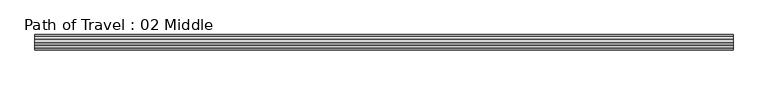
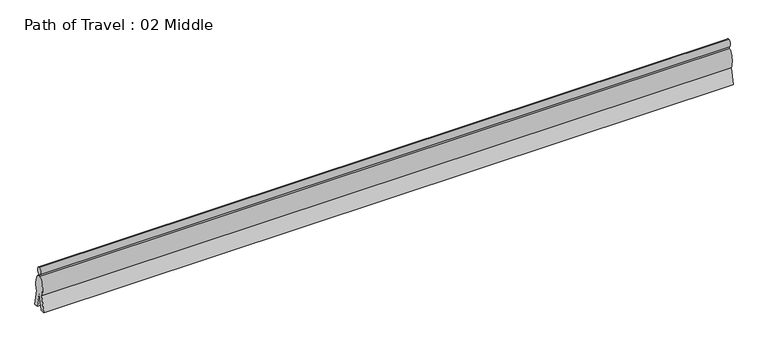
"""IFC4 building model written with IfcOpenShell, lengths in millimetres: proxy geometry, Path of Travel : 02 Middle."""

from ifc_helpers import new_model, si_unit, point, frame, origin, place, context, project, spatial, ellipse_curve, trimmed, source, transform, mapped, element, save
from ifc_brep_helpers import plane_surface, extruded_surface, advanced_brep


def path_of_travel_02_middle_70bd03b1(model_context):
    return source(origin(), model_context, "Body", "AdvancedBrep", [
        advanced_brep(
        [(227.5554837, 0.0, 1727.2), (227.5554837, 42.9018657, 1436.6534209), (227.5554837, 42.9018657, 1363.4763406), (227.5554837, 184.1186263, 643.4144547), (227.5554837, 297.5699544, 0.0), (227.5554837, 145.6574193, 0.0), (227.5554837, 0.0, 584.2), (227.5554837, -145.6574193, 0.0), (227.5554837, -297.5699544, 0.0), (227.5554837, -184.1186263, 643.4144547), (227.5554837, -42.9018657, 1363.4763406), (227.5554837, -42.9018657, 1436.6534209), (27507.1554837, 0.0, 1727.2), (27507.1554837, -42.9018657, 1436.6534209), (27507.1554837, -42.9018657, 1363.4763406), (27507.1554837, -184.1186263, 643.4144547), (27507.1554837, -297.5699544, 0.0), (27507.1554837, -145.6574193, 0.0), (27507.1554837, 0.0, 584.2), (27507.1554837, 145.6574193, 0.0), (27507.1554837, 297.5699544, 0.0), (27507.1554837, 184.1186263, 643.4144547), (27507.1554837, 42.9018657, 1363.4763406), (27507.1554837, 42.9018657, 1436.6534209)],
        [
            (0, 1, ellipse_curve(frame((227.5554837, 0.0, 1574.8), z_axis=(-1.0, 0.0, 0.0), x_axis=(0.0, 0.0, 1.0)), 152.4, 101.6)),
            (1, 2),
            (2, 3, ellipse_curve(frame((227.5554837, 0.0, 914.4), z_axis=(-1.0, 0.0, 0.0), x_axis=(0.0, 0.0, -1.0)), 457.2, 228.6)),
            (3, 4),
            (4, 5),
            (5, 6),
            (6, 7),
            (7, 8),
            (8, 9),
            (9, 10, ellipse_curve(frame((227.5554837, 0.0, 914.4), z_axis=(-1.0, 0.0, 0.0), x_axis=(0.0, 0.0, -1.0)), 457.2, 228.6)),
            (10, 11),
            (11, 0, ellipse_curve(frame((227.5554837, 0.0, 1574.8), z_axis=(-1.0, 0.0, 0.0), x_axis=(0.0, 0.0, 1.0)), 152.4, 101.6)),
            (12, 13, ellipse_curve(frame((27507.1554837, 0.0, 1574.8), z_axis=(1.0, 0.0, 0.0), x_axis=(0.0, 0.0, 1.0)), 152.4, 101.6)),
            (13, 14),
            (14, 15, ellipse_curve(frame((27507.1554837, 0.0, 914.4), z_axis=(1.0, 0.0, 0.0), x_axis=(0.0, 0.0, -1.0)), 457.2, 228.6)),
            (15, 16),
            (16, 17),
            (17, 18),
            (18, 19),
            (19, 20),
            (20, 21),
            (21, 22, ellipse_curve(frame((27507.1554837, 0.0, 914.4), z_axis=(1.0, 0.0, 0.0), x_axis=(0.0, 0.0, -1.0)), 457.2, 228.6)),
            (22, 23),
            (23, 12, ellipse_curve(frame((27507.1554837, 0.0, 1574.8), z_axis=(1.0, 0.0, 0.0), x_axis=(0.0, 0.0, 1.0)), 152.4, 101.6)),
            (0, 12),
            (23, 1),
            (22, 2),
            (21, 3),
            (20, 4),
            (19, 5),
            (18, 6),
            (17, 7),
            (16, 8),
            (15, 9),
            (14, 10),
            (13, 11),
        ],
        [
            plane_surface(frame((227.5554837, 0.0, 0.0), z_axis=(-1.0, 0.0, 0.0), x_axis=(0.0, 0.0, 1.0))),
            plane_surface(frame((27507.1554837, 0.0, 0.0), z_axis=(1.0, 0.0, 0.0), x_axis=(0.0, 0.0, 1.0))),
            extruded_surface(trimmed(ellipse_curve(frame((27507.1554837, 0.0, 1574.8), z_axis=(-1.0, 0.0, 0.0), x_axis=(0.0, 0.0, 1.0)), 152.4, 101.6), [point((27507.1554837, 0.0, 1727.2))], [point((27507.1554837, 42.9018657, 1436.6534209))], True, "CARTESIAN"), (-27279.6, 0.0, 0.0), 27279.6),
            plane_surface(frame((227.5554837, 42.9018657, 1436.6534209), z_axis=(0.0, 1.0, 0.0), x_axis=(1.0, 0.0, 0.0))),
            extruded_surface(trimmed(ellipse_curve(frame((27507.1554837, 0.0, 914.4), z_axis=(-1.0, 0.0, 0.0), x_axis=(0.0, 0.0, -1.0)), 457.2, 228.6), [point((27507.1554837, 42.9018657, 1363.4763406))], [point((27507.1554837, 184.1186263, 643.4144547))], True, "CARTESIAN"), (-27279.6, 0.0, 0.0), 27279.6),
            plane_surface(frame((227.5554837, 184.1186263, 643.4144547), z_axis=(0.0, 0.9848077530122078, 0.17364817766693205), x_axis=(1.0, 0.0, 0.0))),
            plane_surface(frame((227.5554837, 297.5699544, 0.0), z_axis=(0.0, 0.0, -1.0), x_axis=(1.0, 0.0, 0.0))),
            plane_surface(frame((227.5554837, 145.6574193, 0.0), z_axis=(0.0, -0.9702957262760199, -0.2419218955995739), x_axis=(1.0, 0.0, 0.0))),
            plane_surface(frame((227.5554837, 0.0, 584.2), z_axis=(0.0, 0.9702957262759961, -0.24192189559966923), x_axis=(1.0, 0.0, 0.0))),
            plane_surface(frame((227.5554837, -145.6574193, 0.0), z_axis=(0.0, 0.0, -1.0), x_axis=(1.0, 0.0, 0.0))),
            plane_surface(frame((227.5554837, -297.5699544, 0.0), z_axis=(0.0, -0.984807753012208, 0.17364817766693066), x_axis=(1.0, 0.0, 0.0))),
            extruded_surface(trimmed(ellipse_curve(frame((27507.1554837, 0.0, 914.4), z_axis=(-1.0, 0.0, 0.0), x_axis=(0.0, 0.0, -1.0)), 457.2, 228.6), [point((27507.1554837, -184.1186263, 643.4144547))], [point((27507.1554837, -42.9018657, 1363.4763406))], True, "CARTESIAN"), (-27279.6, 0.0, 0.0), 27279.6),
            plane_surface(frame((227.5554837, -42.9018657, 1363.4763406), z_axis=(0.0, -1.0, 0.0), x_axis=(1.0, 0.0, 0.0))),
            extruded_surface(trimmed(ellipse_curve(frame((27507.1554837, 0.0, 1574.8), z_axis=(-1.0, 0.0, 0.0), x_axis=(0.0, 0.0, 1.0)), 152.4, 101.6), [point((27507.1554837, -42.9018657, 1436.6534209))], [point((27507.1554837, 0.0, 1727.2))], True, "CARTESIAN"), (-27279.6, 0.0, 0.0), 27279.6),
        ],
        [
            (0, [[1, 2, 3, 4, 5, 6, 7, 8, 9, 10, 11, 12]]),
            (1, [[13, 14, 15, 16, 17, 18, 19, 20, 21, 22, 23, 24]]),
            (2, [[-1, 25, -24, 26]]),
            (3, [[-2, -26, -23, 27]]),
            (4, [[-3, -27, -22, 28]]),
            (5, [[-4, -28, -21, 29]]),
            (6, [[-5, -29, -20, 30]]),
            (7, [[-6, -30, -19, 31]]),
            (8, [[-7, -31, -18, 32]]),
            (9, [[-8, -32, -17, 33]]),
            (10, [[-9, -33, -16, 34]]),
            (11, [[-10, -34, -15, 35]]),
            (12, [[-11, -35, -14, 36]]),
            (13, [[-12, -36, -13, -25]]),
        ],
    ),
    ])


if __name__ == "__main__":
    model = new_model("IFC4")
    model_context = context("Model", 3, world=origin())
    ifc_project = project(units=[si_unit("LENGTHUNIT", "METRE", prefix="MILLI")], contexts=[model_context])
    site = spatial("IfcSite", under=ifc_project)
    building = spatial("IfcBuilding", under=site)
    placement = place(None, origin())
    path_of_travel_02_middle_shape = path_of_travel_02_middle_70bd03b1(model_context)
    element("IfcBuildingElementProxy", 1, Name="Path of Travel : 02 Middle", ObjectType="Path of Travel : 02 Middle", at=placement, inside=building, context=model_context, shape_type="MappedRepresentation", body=[
        mapped(path_of_travel_02_middle_shape, transform((0.0, 0.0, 0.0), x_axis=(1.0, 0.0, 0.0), y_axis=(0.0, 1.0, 0.0), z_axis=(0.0, 0.0, 1.0))),
    ])
    save(model, "model.ifc")

# Revit data of these elements
# Type "Path of Travel : 02 Middle"
#   Path of Egress [instance default] = 4' - 0"
#   built-in parameter 1001306 [instance default] = 4 (stored number, unit not read)
#   Dot at Start = no
#   Arrow in Middle = yes
#   Arrow at End = no
#   Egress Path = none
# Element 1 (IfcBuildingElementProxy, "Path of Travel : 02 Middle")
#   Path of Egress = 89' - 6"
#   built-in parameter 1001306 = 89.5 (stored number, unit not read)
#   Materials on its faces: "Egress Path Solid"
# Materials
#   "Egress Path Solid": class "Unassigned", colour RGB 255 128 64, transparency 0.75, Comments = "Rendering appearance not upgraded "
